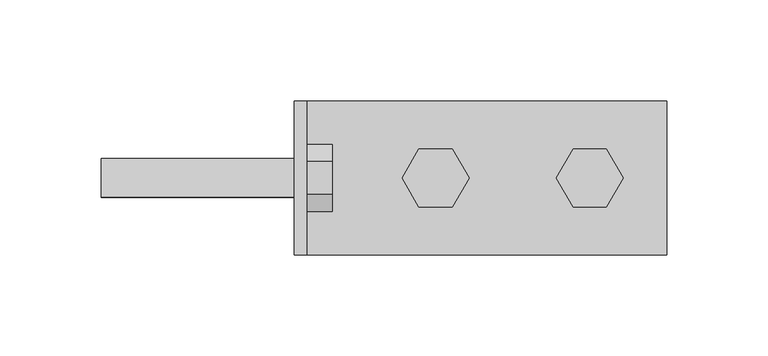
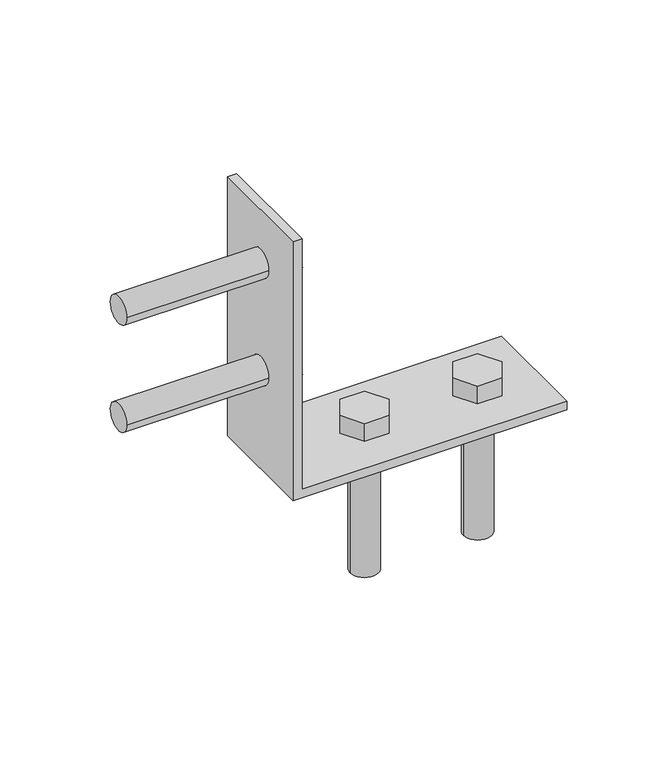
"""IFC4 building model written with IfcOpenShell, lengths in millimetres: fastener geometry, SIMPSON - HLPC/HLGPC Heavy Angles and Gussets : SIMPSON -HL73 - 3 X 7.25 - .75 Bolt - HDG."""

import ifcopenshell
import ifcopenshell.guid

model = None  # the IFC model being written
_history = None  # IfcOwnerHistory: only IFC2X3 demands one
_inside = {}  # id of a spatial element -> (the spatial element, [elements in it])
_under = {}  # id of a project, library or spatial element -> (it, [spatial elements below it])
_declared = {}  # id of a project -> (the project, [libraries it declares])
_typed = {}  # id of a type object -> (the type object, [elements of that type])
_made_of = {}  # id of a material, layer set ... -> (it, [elements and type objects made of it])


def new_model(schema):
    """Start an empty IFC model of exactly this schema.

    Asked for "IFC4X3", IfcOpenShell would pick the latest addendum, in which some entities
    have other attributes; the version numbers below select the first issue.
    IFC2X3 requires an IfcOwnerHistory on every rooted entity: one is made here for all.
    """
    global model, _history
    if schema == "IFC4X3":
        model = ifcopenshell.file(schema_version=(4, 3, 0, 0))
    else:
        model = ifcopenshell.file(schema=schema)
    _inside.clear()
    _under.clear()
    _declared.clear()
    _typed.clear()
    _made_of.clear()
    _history = None
    if model.schema == "IFC2X3":
        org = make("IfcOrganization", Name="unknown")
        user = make(
            "IfcPersonAndOrganization",
            ThePerson=make("IfcPerson", FamilyName="unknown"),
            TheOrganization=org,
        )
        app = make(
            "IfcApplication",
            ApplicationDeveloper=org,
            Version="unknown",
            ApplicationFullName="unknown",
            ApplicationIdentifier="unknown",
        )
        _history = make(
            "IfcOwnerHistory",
            OwningUser=user,
            OwningApplication=app,
            ChangeAction="ADDED",
            CreationDate=0,
        )
    return model


def make(cls, **values):
    """One entity of the class cls with the attributes given. An attribute that is None is left unset."""
    return model.create_entity(
        cls, **{name: value for name, value in values.items() if value is not None}
    )


def rooted(cls, **values):
    """An entity with a GlobalId (a new one), such as an element, a storey or a relation."""
    return make(cls, GlobalId=ifcopenshell.guid.new(), OwnerHistory=_history, **values)


def si_unit(unit_type, name, prefix=None):
    """IfcSIUnit, for example si_unit("LENGTHUNIT", "METRE", prefix="MILLI")."""
    return make("IfcSIUnit", UnitType=unit_type, Prefix=prefix, Name=name)


def assignment(units):
    """IfcUnitAssignment: the units of a project."""
    return None if units is None else make("IfcUnitAssignment", Units=units)


def point(xyz):
    """IfcCartesianPoint."""
    return None if xyz is None else make("IfcCartesianPoint", Coordinates=xyz)


def direction(xyz):
    """IfcDirection."""
    return None if xyz is None else make("IfcDirection", DirectionRatios=xyz)


def frame(location, z_axis=None, x_axis=None):
    """IfcAxis2Placement3D, a coordinate frame: its origin and axes. An axis left out is left unset."""
    return make(
        "IfcAxis2Placement3D",
        Location=point(location),
        Axis=direction(z_axis),
        RefDirection=direction(x_axis),
    )


def frame_2d(location, x_axis=None):
    """IfcAxis2Placement2D, a coordinate frame in the plane: its origin and x axis."""
    return make(
        "IfcAxis2Placement2D", Location=point(location), RefDirection=direction(x_axis)
    )


def origin():
    """The frame at (0, 0, 0) with its axes left unset."""
    return frame((0.0, 0.0, 0.0))


def place(relative_to, where):
    """IfcLocalPlacement: puts the frame where relative to a parent placement (None: the world)."""
    return make(
        "IfcLocalPlacement", PlacementRelTo=relative_to, RelativePlacement=where
    )


def context(
    kind, dimensions, precision=None, world=None, true_north=None, identifier=None
):
    """IfcGeometricRepresentationContext, for example the 3D "Model" context."""
    return make(
        "IfcGeometricRepresentationContext",
        ContextIdentifier=identifier,
        ContextType=kind,
        CoordinateSpaceDimension=dimensions,
        Precision=precision,
        WorldCoordinateSystem=world,
        TrueNorth=true_north,
    )


def project(units=None, contexts=None):
    """IfcProject with its units and contexts."""
    return rooted(
        "IfcProject",
        Name="project",
        RepresentationContexts=contexts,
        UnitsInContext=assignment(units),
    )


def spatial(cls, under=None, at=None, **own):
    """A site, building, storey or space (cls), placed at a placement, below another one or the project."""
    s = rooted(cls, ObjectPlacement=at, **own)
    if under is not None:
        _under.setdefault(under.id(), (under, []))[1].append(s)
    return s


def polyline(points):
    """IfcPolyline through the points."""
    return make("IfcPolyline", Points=[point(p) for p in points])


def circle_curve(where, radius):
    """IfcCircle in the frame where."""
    return make("IfcCircle", Position=where, Radius=radius)


def trimmed(basis, trim1, trim2, sense, master):
    """IfcTrimmedCurve: the piece of a basis curve between two trims."""
    return make(
        "IfcTrimmedCurve",
        BasisCurve=basis,
        Trim1=trim1,
        Trim2=trim2,
        SenseAgreement=sense,
        MasterRepresentation=master,
    )


def segment(curve, same_sense, transition):
    """IfcCompositeCurveSegment."""
    return make(
        "IfcCompositeCurveSegment",
        Transition=transition,
        SameSense=same_sense,
        ParentCurve=curve,
    )


def composite_curve(segments, self_intersect=None):
    """IfcCompositeCurve: segments joined end to end."""
    return make("IfcCompositeCurve", Segments=segments, SelfIntersect=self_intersect)


def outline(outer, holes=None, kind="AREA"):
    """IfcArbitraryClosedProfileDef: a profile drawn as a closed curve; with holes, ...WithVoids."""
    if holes is None:
        return make("IfcArbitraryClosedProfileDef", ProfileType=kind, OuterCurve=outer)
    return make(
        "IfcArbitraryProfileDefWithVoids",
        ProfileType=kind,
        OuterCurve=outer,
        InnerCurves=holes,
    )


def extrude(swept, where, along, depth):
    """IfcExtrudedAreaSolid: the profile swept, set in the frame where, extruded along a direction by depth."""
    return make(
        "IfcExtrudedAreaSolid",
        SweptArea=swept,
        Position=where,
        ExtrudedDirection=direction(along),
        Depth=depth,
    )


def shape(context_of_items, identifier, shape_type, items):
    """IfcShapeRepresentation: the items that make up one representation, for example the "Body"."""
    return make(
        "IfcShapeRepresentation",
        ContextOfItems=context_of_items,
        RepresentationIdentifier=identifier,
        RepresentationType=shape_type,
        Items=items,
    )


def source(mapping_origin, context_of_items, identifier, shape_type, items):
    """IfcRepresentationMap: a shape defined once, which mapped items show again and again."""
    return make(
        "IfcRepresentationMap",
        MappingOrigin=mapping_origin,
        MappedRepresentation=shape(context_of_items, identifier, shape_type, items),
    )


def transform(
    local_origin,
    x_axis=None,
    y_axis=None,
    z_axis=None,
    scale=None,
    scale2=None,
    scale3=None,
    uniform=True,
):
    """IfcCartesianTransformationOperator3D, or its non-uniform kind. x_axis, y_axis, z_axis: its Axis1, 2, 3."""
    if uniform:
        return make(
            "IfcCartesianTransformationOperator3D",
            Axis1=direction(x_axis),
            Axis2=direction(y_axis),
            LocalOrigin=point(local_origin),
            Scale=scale,
            Axis3=direction(z_axis),
        )
    return make(
        "IfcCartesianTransformationOperator3DnonUniform",
        Axis1=direction(x_axis),
        Axis2=direction(y_axis),
        LocalOrigin=point(local_origin),
        Scale=scale,
        Axis3=direction(z_axis),
        Scale2=scale2,
        Scale3=scale3,
    )


def mapped(mapping_source, mapping_target):
    """IfcMappedItem: shows the shape of a source again, moved by a transform."""
    return make(
        "IfcMappedItem", MappingSource=mapping_source, MappingTarget=mapping_target
    )


def made_of(thing, what):
    """Note that an element or type object is made of a material, layer set ...; save() writes the relation."""
    if what is not None:
        _made_of.setdefault(what.id(), (what, []))[1].append(thing)
    return thing


def element(
    cls,
    number,
    at=None,
    inside=None,
    cuts=None,
    type_object=None,
    material=None,
    context=None,
    identifier="Body",
    shape_type=None,
    held_by="IfcProductDefinitionShape",
    body=None,
    shapes=None,
    **own,
):
    """One element of the class cls, such as IfcWall. Its Tag is "e" and its number.

    at: its placement. inside: the storey or other place that contains it. cuts: it is an
    opening in that element (IfcRelVoidsElement). A single representation is given by context,
    identifier, shape_type and body (its items); several are given by shapes. held_by: the class
    of the entity that holds the representations. save() writes the other relations.
    """
    e = rooted(cls, Tag="e%d" % number, ObjectPlacement=at, **own)
    if body is not None:
        shapes = [shape(context, identifier, shape_type, body)]
    if shapes is not None:
        e.Representation = make(held_by, Representations=shapes)
    if inside is not None:
        _inside.setdefault(inside.id(), (inside, []))[1].append(e)
    if cuts is not None:
        rooted(
            "IfcRelVoidsElement", RelatingBuildingElement=cuts, RelatedOpeningElement=e
        )
    if type_object is not None:
        _typed.setdefault(type_object.id(), (type_object, []))[1].append(e)
    return made_of(e, material)


def aggregate(whole, parts):
    """IfcRelAggregates: a whole, such as a stair, and the parts it consists of."""
    return rooted("IfcRelAggregates", RelatingObject=whole, RelatedObjects=parts)


def save(model, path):
    """Write the relations noted so far, then the file.

    IfcRelAggregates (storeys below a building ...), IfcRelContainedInSpatialStructure (elements
    in a storey), IfcRelDefinesByType, IfcRelAssociatesMaterial and IfcRelDeclares: one each for
    every whole, place, type object, material and project.
    """
    for whole, parts in _under.values():
        aggregate(whole, parts)
    for where, things in _inside.values():
        rooted(
            "IfcRelContainedInSpatialStructure",
            RelatedElements=things,
            RelatingStructure=where,
        )
    for kind, things in _typed.values():
        rooted("IfcRelDefinesByType", RelatedObjects=things, RelatingType=kind)
    for what, things in _made_of.values():
        rooted("IfcRelAssociatesMaterial", RelatedObjects=things, RelatingMaterial=what)
    for by, libraries in _declared.values():
        rooted("IfcRelDeclares", RelatingContext=by, RelatedDefinitions=libraries)
    model.write(path)


def plane_surface(at):
    """IfcPlane: the flat surface through the origin of the frame at, square to its z axis."""
    return make("IfcPlane", Position=at)


def revolved_surface(curve, axis_point, axis_direction):
    """IfcSurfaceOfRevolution: the curve turned about the line through axis_point along axis_direction."""
    return make(
        "IfcSurfaceOfRevolution",
        SweptCurve=make("IfcArbitraryOpenProfileDef", ProfileType="CURVE", Curve=curve),
        AxisPosition=make("IfcAxis1Placement", Location=point(axis_point), Axis=direction(axis_direction)),
    )


def advanced_brep(points, edges, surfaces, faces):
    """IfcAdvancedBrep: a solid bounded by faces that lie on surfaces and meet in shared edges.

    An edge is (start, end): straight between two places in points (the first is 0);
    or (start, end, curve); or (start, end, curve, False) where it runs against its curve.
    A face is (place in surfaces, loops), or (place, loops, False) where it looks against
    its surface's normal. A loop lists edges by number (the first is 1), with a minus sign
    where the edge is run from its end to its start. The first loop is the outer one.
    """
    corners = [point(p) for p in points]
    vertices = [make("IfcVertexPoint", VertexGeometry=c) for c in corners]
    made = []
    for start, end, *more in edges:
        made.append(
            make(
                "IfcEdgeCurve",
                EdgeStart=vertices[start],
                EdgeEnd=vertices[end],
                EdgeGeometry=more[0] if more else make("IfcPolyline", Points=[corners[start], corners[end]]),
                SameSense=more[1] if len(more) > 1 else True,
            )
        )
    hull = []
    for where, loops, *sense in faces:
        bounds = []
        for j, loop in enumerate(loops):
            ring = [make("IfcOrientedEdge", EdgeElement=made[abs(k) - 1], Orientation=k > 0) for k in loop]
            bounds.append(
                make(
                    "IfcFaceOuterBound" if j == 0 else "IfcFaceBound",
                    Bound=make("IfcEdgeLoop", EdgeList=ring),
                    Orientation=True,
                )
            )
        hull.append(make("IfcAdvancedFace", Bounds=bounds, FaceSurface=surfaces[where], SameSense=sense[0] if sense else True))
    return make("IfcAdvancedBrep", Outer=make("IfcClosedShell", CfsFaces=hull))


def fastener_5e5bee1c(model_context):
    return source(origin(), model_context, "Body", "SolidModel", [
        extrude(outline(composite_curve([segment(trimmed(circle_curve(frame_2d((0.0, 69.85)), 9.525), [point((9.525, 69.85))], [point((-9.525, 69.85))], False, "CARTESIAN"), True, "CONTINUOUS"), segment(trimmed(circle_curve(frame_2d((0.0, 69.85)), 9.525), [point((-9.525, 69.85))], [point((9.525, 69.85))], False, "CARTESIAN"), True, "CONTINUOUS")], self_intersect=False)), frame((-95.5476562, 0.0, 0.0), z_axis=(1.0, 0.0, 0.0), x_axis=(0.0, 1.0, 0.0)), (0.0, 0.0, 1.0), 101.6),
        extrude(outline(polyline([(16.4977839, 69.85), (8.248892, 55.5625), (-8.248892, 55.5625), (-16.4977839, 69.85), (-8.248892, 84.1375), (8.248892, 84.1375), (16.4977839, 69.85)])), frame((6.0523438, 0.0, 0.0), z_axis=(1.0, 0.0, 0.0), x_axis=(0.0, 1.0, 0.0)), (0.0, 0.0, 1.0), 12.7),
        extrude(outline(composite_curve([segment(trimmed(circle_curve(frame_2d((0.0, 146.05)), 9.525), [point((9.525, 146.05))], [point((-9.525, 146.05))], False, "CARTESIAN"), True, "CONTINUOUS"), segment(trimmed(circle_curve(frame_2d((0.0, 146.05)), 9.525), [point((-9.525, 146.05))], [point((9.525, 146.05))], False, "CARTESIAN"), True, "CONTINUOUS")], self_intersect=False)), frame((-95.5476562, 0.0, 0.0), z_axis=(1.0, 0.0, 0.0), x_axis=(0.0, 1.0, 0.0)), (0.0, 0.0, 1.0), 101.6),
        extrude(outline(polyline([(16.4977839, 146.05), (8.248892, 131.7625), (-8.248892, 131.7625), (-16.4977839, 146.05), (-8.248892, 160.3375), (8.248892, 160.3375), (16.4977839, 146.05)])), frame((6.0523438, 0.0, 0.0), z_axis=(1.0, 0.0, 0.0), x_axis=(0.0, 1.0, 0.0)), (0.0, 0.0, 1.0), 12.7),
        extrude(outline(composite_curve([segment(trimmed(circle_curve(frame_2d((146.05, 0.0)), 9.525), [point((136.525, 0.0))], [point((155.575, 0.0))], False, "CARTESIAN"), True, "CONTINUOUS"), segment(trimmed(circle_curve(frame_2d((146.05, 0.0)), 9.525), [point((155.575, 0.0))], [point((136.525, 0.0))], False, "CARTESIAN"), True, "CONTINUOUS")], self_intersect=False)), frame((0.0, 0.0, -95.5476563), z_axis=(0.0, 0.0, 1.0), x_axis=(1.0, 0.0, 0.0)), (0.0, 0.0, 1.0), 101.6),
        extrude(outline(polyline([(129.5522161, 0.0), (137.801108, 14.2875), (154.298892, 14.2875), (162.5477839, 0.0), (154.298892, -14.2875), (137.801108, -14.2875), (129.5522161, 0.0)])), frame((0.0, 0.0, 6.0523437), z_axis=(0.0, 0.0, 1.0), x_axis=(1.0, 0.0, 0.0)), (0.0, 0.0, 1.0), 12.7),
        extrude(outline(composite_curve([segment(trimmed(circle_curve(frame_2d((69.85, 0.0)), 9.525), [point((60.325, 0.0))], [point((79.375, 0.0))], False, "CARTESIAN"), True, "CONTINUOUS"), segment(trimmed(circle_curve(frame_2d((69.85, 0.0)), 9.525), [point((79.375, 0.0))], [point((60.325, 0.0))], False, "CARTESIAN"), True, "CONTINUOUS")], self_intersect=False)), frame((0.0, 0.0, -95.5476563), z_axis=(0.0, 0.0, 1.0), x_axis=(1.0, 0.0, 0.0)), (0.0, 0.0, 1.0), 101.6),
        extrude(outline(polyline([(53.3522161, 0.0), (61.601108, 14.2875), (78.098892, 14.2875), (86.3477839, 0.0), (78.098892, -14.2875), (61.601108, -14.2875), (53.3522161, 0.0)])), frame((0.0, 0.0, 6.0523437), z_axis=(0.0, 0.0, 1.0), x_axis=(1.0, 0.0, 0.0)), (0.0, 0.0, 1.0), 12.7),
        advanced_brep(
        [(6.0523438, -38.1, 184.15), (6.0523438, -38.1, 6.0523437), (6.0523438, 38.1, 6.0523437), (6.0523438, 38.1, 184.15), (6.0523438, -9.525, 69.85), (6.0523438, 9.525, 69.85), (6.0523438, -9.525, 146.05), (6.0523438, 9.525, 146.05), (0.0, 38.1, 184.15), (0.0, 38.1, 0.0), (0.0, -38.1, 0.0), (0.0, -38.1, 184.15), (0.0, 9.525, 69.85), (0.0, -9.525, 69.85), (0.0, 9.525, 146.05), (0.0, -9.525, 146.05), (184.15, 38.1, 6.0523437), (184.15, 38.1, 0.0), (184.15, -38.1, 0.0), (184.15, -38.1, 6.0523437), (79.375, 0.0, 6.0523437), (60.325, 0.0, 6.0523437), (155.575, 0.0, 6.0523437), (136.525, 0.0, 6.0523437), (60.325, 0.0, 0.0), (79.375, 0.0, 0.0), (136.525, 0.0, 0.0), (155.575, 0.0, 0.0)],
        [
            (0, 1),
            (1, 2),
            (2, 3),
            (3, 0),
            (4, 5, circle_curve(frame((6.0523438, 0.0, 69.85), z_axis=(-1.0, 0.0, 0.0), x_axis=(0.0, -1.0, 0.0)), 9.525)),
            (5, 4, circle_curve(frame((6.0523438, 0.0, 69.85), z_axis=(-1.0, 0.0, 0.0), x_axis=(0.0, -1.0, 0.0)), 9.525)),
            (6, 7, circle_curve(frame((6.0523438, 0.0, 146.05), z_axis=(-1.0, 0.0, 0.0), x_axis=(0.0, -1.0, 0.0)), 9.525)),
            (7, 6, circle_curve(frame((6.0523438, 0.0, 146.05), z_axis=(-1.0, 0.0, 0.0), x_axis=(0.0, -1.0, 0.0)), 9.525)),
            (8, 9),
            (9, 10),
            (10, 11),
            (11, 8),
            (12, 13, circle_curve(frame((0.0, 0.0, 69.85), z_axis=(1.0, 0.0, 0.0), x_axis=(0.0, -1.0, 0.0)), 9.525)),
            (13, 12, circle_curve(frame((0.0, 0.0, 69.85), z_axis=(1.0, 0.0, 0.0), x_axis=(0.0, -1.0, 0.0)), 9.525)),
            (14, 15, circle_curve(frame((0.0, 0.0, 146.05), z_axis=(1.0, 0.0, 0.0), x_axis=(0.0, -1.0, 0.0)), 9.525)),
            (15, 14, circle_curve(frame((0.0, 0.0, 146.05), z_axis=(1.0, 0.0, 0.0), x_axis=(0.0, -1.0, 0.0)), 9.525)),
            (3, 8),
            (11, 0),
            (2, 16),
            (16, 17),
            (17, 9),
            (10, 18),
            (18, 19),
            (19, 1),
            (19, 16),
            (20, 21, circle_curve(frame((69.85, 0.0, 6.0523437), z_axis=(0.0, 0.0, -1.0), x_axis=(1.0, 0.0, 0.0)), 9.525)),
            (21, 20, circle_curve(frame((69.85, 0.0, 6.0523437), z_axis=(0.0, 0.0, -1.0), x_axis=(1.0, 0.0, 0.0)), 9.525)),
            (22, 23, circle_curve(frame((146.05, 0.0, 6.0523437), z_axis=(0.0, 0.0, -1.0), x_axis=(1.0, 0.0, 0.0)), 9.525)),
            (23, 22, circle_curve(frame((146.05, 0.0, 6.0523437), z_axis=(0.0, 0.0, -1.0), x_axis=(1.0, 0.0, 0.0)), 9.525)),
            (17, 18),
            (24, 25, circle_curve(frame((69.85, 0.0, 0.0), z_axis=(0.0, 0.0, 1.0), x_axis=(1.0, 0.0, 0.0)), 9.525)),
            (25, 24, circle_curve(frame((69.85, 0.0, 0.0), z_axis=(0.0, 0.0, 1.0), x_axis=(1.0, 0.0, 0.0)), 9.525)),
            (26, 27, circle_curve(frame((146.05, 0.0, 0.0), z_axis=(0.0, 0.0, 1.0), x_axis=(1.0, 0.0, 0.0)), 9.525)),
            (27, 26, circle_curve(frame((146.05, 0.0, 0.0), z_axis=(0.0, 0.0, 1.0), x_axis=(1.0, 0.0, 0.0)), 9.525)),
            (21, 24),
            (25, 20),
            (23, 26),
            (27, 22),
            (5, 12),
            (13, 4),
            (7, 14),
            (15, 6),
        ],
        [
            plane_surface(frame((6.0523438, 38.1, 184.15), z_axis=(1.0, 0.0, 0.0), x_axis=(0.0, 1.0, 0.0))),
            plane_surface(frame((0.0, 38.1, 184.15), z_axis=(-1.0, 0.0, 0.0), x_axis=(0.0, -1.0, 0.0))),
            plane_surface(frame((6.0523438, -38.1, 184.15), z_axis=(0.0, 0.0, 1.0), x_axis=(-1.0, 0.0, 0.0))),
            plane_surface(frame((6.0523438, 38.1, 184.15), z_axis=(0.0, 1.0, 0.0), x_axis=(-1.0, 0.0, 0.0))),
            plane_surface(frame((6.0523438, -38.1, 6.0523437), z_axis=(0.0, -1.0, 0.0), x_axis=(-1.0, 0.0, 0.0))),
            plane_surface(frame((0.0, -38.1, 6.0523437), z_axis=(0.0, 0.0, 1.0), x_axis=(-1.0, 0.0, 0.0))),
            plane_surface(frame((0.0, -38.1, 0.0), z_axis=(0.0, 0.0, -1.0), x_axis=(1.0, 0.0, 0.0))),
            plane_surface(frame((184.15, 38.1, 6.0523437), z_axis=(1.0, 0.0, 0.0), x_axis=(0.0, 0.0, -1.0))),
            revolved_surface(polyline([(79.375, 0.0, 6.0523437), (79.375, 0.0, 0.0)]), (69.85, 0.0, 0.0), (0.0, 0.0, 1.0)),
            revolved_surface(polyline([(155.57500000000002, 0.0, 6.0523437), (155.57500000000002, 0.0, 0.0)]), (146.05, 0.0, 0.0), (0.0, 0.0, 1.0)),
            revolved_surface(polyline([(6.0523438, -9.525, 69.85), (0.0, -9.525, 69.85)]), (0.0, 0.0, 69.85), (1.0, 0.0, 0.0)),
            revolved_surface(polyline([(6.0523438, -9.525, 146.05), (0.0, -9.525, 146.05)]), (0.0, 0.0, 146.05), (1.0, 0.0, 0.0)),
        ],
        [
            (0, [[1, 2, 3, 4], [5, 6], [7, 8]]),
            (1, [[9, 10, 11, 12], [13, 14], [15, 16]]),
            (2, [[17, -12, 18, -4]]),
            (3, [[19, 20, 21, -9, -17, -3]]),
            (4, [[-18, -11, 22, 23, 24, -1]]),
            (5, [[-19, -2, -24, 25], [26, 27], [28, 29]]),
            (6, [[-22, -10, -21, 30], [31, 32], [33, 34]]),
            (7, [[-23, -30, -20, -25]]),
            (8, [[-27, 35, -32, 36]]),
            (8, [[-31, -35, -26, -36]]),
            (9, [[-29, 37, -34, 38]]),
            (9, [[-33, -37, -28, -38]]),
            (10, [[-6, 39, -14, 40]]),
            (10, [[-13, -39, -5, -40]]),
            (11, [[-8, 41, -16, 42]]),
            (11, [[-15, -41, -7, -42]]),
        ],
    ),
    ])


if __name__ == "__main__":
    model = new_model("IFC4")
    model_context = context("Model", 3, world=origin())
    ifc_project = project(units=[si_unit("LENGTHUNIT", "METRE", prefix="MILLI")], contexts=[model_context])
    site = spatial("IfcSite", under=ifc_project)
    building = spatial("IfcBuilding", under=site)
    placement = place(None, origin())
    fastener_shape = fastener_5e5bee1c(model_context)
    element("IfcFastener", 1, ObjectType="SIMPSON - HLPC/HLGPC Heavy Angles and Gussets : SIMPSON -HL73 - 3 X 7.25 - .75 Bolt - HDG", at=placement, inside=building, context=model_context, shape_type="MappedRepresentation", body=[
        mapped(fastener_shape, transform((0.0, 0.0, 0.0), x_axis=(1.0, 0.0, 0.0), y_axis=(0.0, 1.0, 0.0), z_axis=(0.0, 0.0, 1.0))),
    ])
    save(model, "model.ifc")

# Revit data of these elements
# Type "SIMPSON - HLPC/HLGPC Heavy Angles and Gussets : SIMPSON -HL73 - 3 X 7.25 - .75 Bolt - HDG"
#   URL = "https://www.strongtie.com/classiccollection_architecturalproductsgroup/hlpc-hlgpc_productgroup_wcc/p/hlpc.hlgpc"
#   L = 0' - 3"
#   Hole Radius = 0' - 0 3/8"
#   D4 = 0' - 3"
#   D2 = 0' - 5"
#   D1 = 0' - 1 1/2"
#   D3 = 0' - 2 3/4"
#   Ga. = 0' - 0 61/256"
#   W1 & W2 = 0' - 7 1/4"
#   Default Elevation = 4' - 0"
#   Bolt Visibility - 3B = no
#   Bolt Visibility - 3A = no
#   Bolt Visibility - 2B = no
#   Bolt Visibility - 2A = no
#   Bolt Visibility - 1B = yes
#   Bolt Visibility - 1A = yes
#   Bolt Visibility = yes
#   Bolt Size = element 1298415
# Element 1 (IfcFastener, "SIMPSON - HLPC/HLGPC Heavy Angles and Gussets : SIMPSON -HL73 - 3 X 7.25 - .75 Bolt - HDG")
#   Materials on its faces: "1\" GALV. LAG BOLT (LENGTH = 1/2\" SHY OF GLULAM DEPTH) -  (GALV. THRU BOLT IF PLATE ON OPP. SIDE OF STRUCT MEMBER)"
# Materials
#   "1\" GALV. LAG BOLT (LENGTH = 1/2\" SHY OF GLULAM DEPTH) -  (GALV. THRU BOLT IF PLATE ON OPP. SIDE OF STRUCT MEMBER)": class "Generic", colour RGB 120 120 120, transparency 0, Cost = 0
